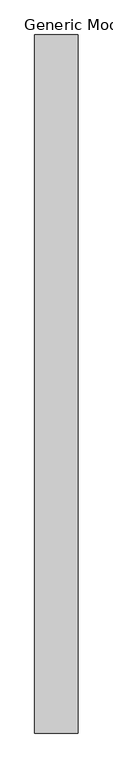
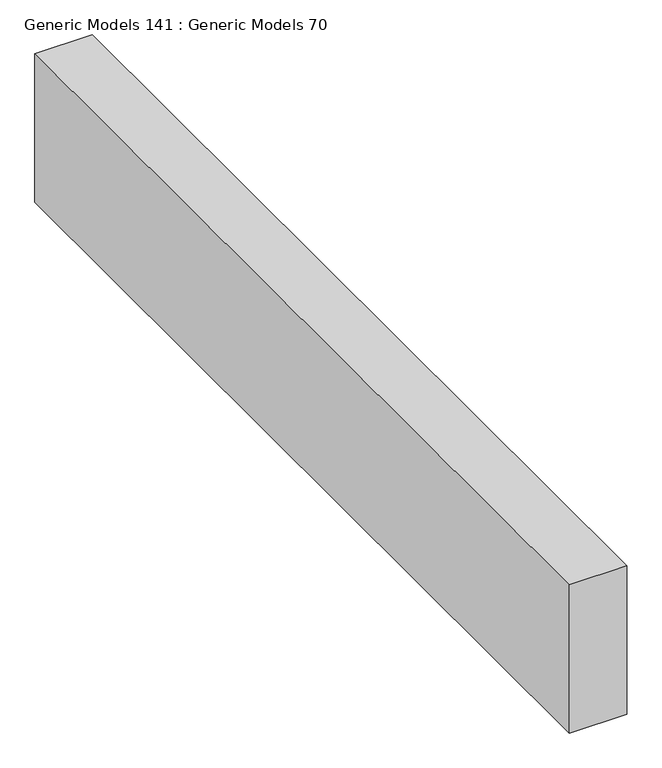
"""IFC4 building model written with IfcOpenShell, lengths in millimetres: proxy geometry, Generic Models 141 : Generic Models 70."""

from ifc_helpers import new_model, si_unit, frame, origin, place, context, project, spatial, polyline, outline, extrude, source, transform, mapped, element, save


def generic_models_141_generic_models_70_328457f7(model_context):
    return source(origin(), model_context, "Body", "SweptSolid", [
        extrude(outline(polyline([(32200.8585525, 30688.6156612), (32200.8585525, 28437.6872112), (32061.1585525, 28437.6872112), (32061.1585525, 30688.6156612), (32200.8585525, 30688.6156612)])), frame((0.0, 0.0, 268757.4), z_axis=(0.0, 0.0, 1.0), x_axis=(1.0, 0.0, 0.0)), (0.0, 0.0, 1.0), 381.0),
    ])


if __name__ == "__main__":
    model = new_model("IFC4")
    model_context = context("Model", 3, world=origin())
    ifc_project = project(units=[si_unit("LENGTHUNIT", "METRE", prefix="MILLI")], contexts=[model_context])
    site = spatial("IfcSite", under=ifc_project)
    building = spatial("IfcBuilding", under=site)
    placement = place(None, origin())
    generic_models_141_generic_models_70_shape = generic_models_141_generic_models_70_328457f7(model_context)
    element("IfcBuildingElementProxy", 1, Name="Generic Models 141 : Generic Models 70", ObjectType="Generic Models 141 : Generic Models 70", at=placement, inside=building, context=model_context, shape_type="MappedRepresentation", body=[
        mapped(generic_models_141_generic_models_70_shape, transform((0.0, 0.0, 0.0), x_axis=(1.0, 0.0, 0.0), y_axis=(0.0, 1.0, 0.0), z_axis=(0.0, 0.0, 1.0))),
    ])
    save(model, "model.ifc")

# Revit data of these elements
# Element 1 (IfcBuildingElementProxy, "Generic Models 141 : Generic Models 70")
#   Materials on its faces: "3 1/2\" x 15\" GLUELAM BEAM"
# Materials
#   "3 1/2\" x 15\" GLUELAM BEAM": class "Wood", colour RGB 214 169 150, transparency 0, Description = "Pinus Echinata", Cost = 0
